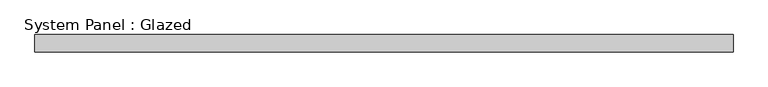
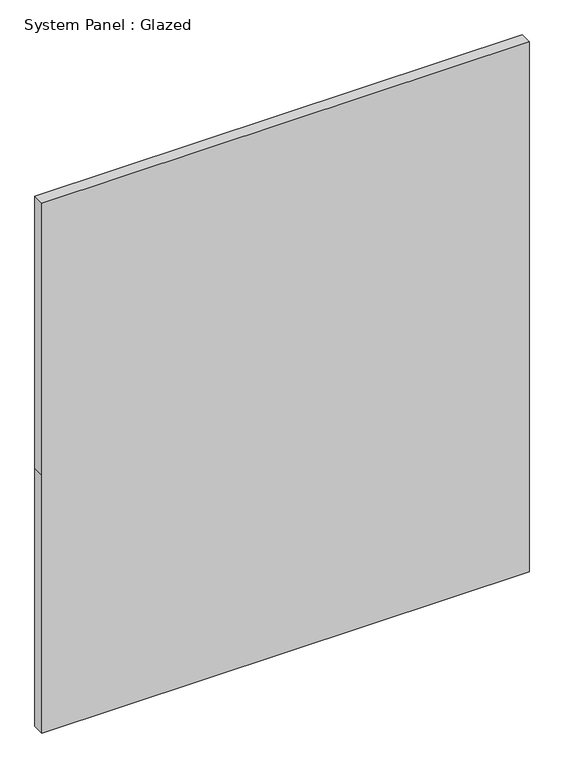
"""IFC4 building model written with IfcOpenShell, lengths in millimetres: plate geometry, System Panel : Glazed."""

import ifcopenshell
import ifcopenshell.guid

model = None  # the IFC model being written
_history = None  # IfcOwnerHistory: only IFC2X3 demands one
_inside = {}  # id of a spatial element -> (the spatial element, [elements in it])
_under = {}  # id of a project, library or spatial element -> (it, [spatial elements below it])
_declared = {}  # id of a project -> (the project, [libraries it declares])
_typed = {}  # id of a type object -> (the type object, [elements of that type])
_made_of = {}  # id of a material, layer set ... -> (it, [elements and type objects made of it])


def new_model(schema):
    """Start an empty IFC model of exactly this schema.

    Asked for "IFC4X3", IfcOpenShell would pick the latest addendum, in which some entities
    have other attributes; the version numbers below select the first issue.
    IFC2X3 requires an IfcOwnerHistory on every rooted entity: one is made here for all.
    """
    global model, _history
    if schema == "IFC4X3":
        model = ifcopenshell.file(schema_version=(4, 3, 0, 0))
    else:
        model = ifcopenshell.file(schema=schema)
    _inside.clear()
    _under.clear()
    _declared.clear()
    _typed.clear()
    _made_of.clear()
    _history = None
    if model.schema == "IFC2X3":
        org = make("IfcOrganization", Name="unknown")
        user = make(
            "IfcPersonAndOrganization",
            ThePerson=make("IfcPerson", FamilyName="unknown"),
            TheOrganization=org,
        )
        app = make(
            "IfcApplication",
            ApplicationDeveloper=org,
            Version="unknown",
            ApplicationFullName="unknown",
            ApplicationIdentifier="unknown",
        )
        _history = make(
            "IfcOwnerHistory",
            OwningUser=user,
            OwningApplication=app,
            ChangeAction="ADDED",
            CreationDate=0,
        )
    return model


def make(cls, **values):
    """One entity of the class cls with the attributes given. An attribute that is None is left unset."""
    return model.create_entity(
        cls, **{name: value for name, value in values.items() if value is not None}
    )


def rooted(cls, **values):
    """An entity with a GlobalId (a new one), such as an element, a storey or a relation."""
    return make(cls, GlobalId=ifcopenshell.guid.new(), OwnerHistory=_history, **values)


def si_unit(unit_type, name, prefix=None):
    """IfcSIUnit, for example si_unit("LENGTHUNIT", "METRE", prefix="MILLI")."""
    return make("IfcSIUnit", UnitType=unit_type, Prefix=prefix, Name=name)


def assignment(units):
    """IfcUnitAssignment: the units of a project."""
    return None if units is None else make("IfcUnitAssignment", Units=units)


def point(xyz):
    """IfcCartesianPoint."""
    return None if xyz is None else make("IfcCartesianPoint", Coordinates=xyz)


def direction(xyz):
    """IfcDirection."""
    return None if xyz is None else make("IfcDirection", DirectionRatios=xyz)


def frame(location, z_axis=None, x_axis=None):
    """IfcAxis2Placement3D, a coordinate frame: its origin and axes. An axis left out is left unset."""
    return make(
        "IfcAxis2Placement3D",
        Location=point(location),
        Axis=direction(z_axis),
        RefDirection=direction(x_axis),
    )


def origin():
    """The frame at (0, 0, 0) with its axes left unset."""
    return frame((0.0, 0.0, 0.0))


def place(relative_to, where):
    """IfcLocalPlacement: puts the frame where relative to a parent placement (None: the world)."""
    return make(
        "IfcLocalPlacement", PlacementRelTo=relative_to, RelativePlacement=where
    )


def context(
    kind, dimensions, precision=None, world=None, true_north=None, identifier=None
):
    """IfcGeometricRepresentationContext, for example the 3D "Model" context."""
    return make(
        "IfcGeometricRepresentationContext",
        ContextIdentifier=identifier,
        ContextType=kind,
        CoordinateSpaceDimension=dimensions,
        Precision=precision,
        WorldCoordinateSystem=world,
        TrueNorth=true_north,
    )


def project(units=None, contexts=None):
    """IfcProject with its units and contexts."""
    return rooted(
        "IfcProject",
        Name="project",
        RepresentationContexts=contexts,
        UnitsInContext=assignment(units),
    )


def spatial(cls, under=None, at=None, **own):
    """A site, building, storey or space (cls), placed at a placement, below another one or the project."""
    s = rooted(cls, ObjectPlacement=at, **own)
    if under is not None:
        _under.setdefault(under.id(), (under, []))[1].append(s)
    return s


def polyline(points):
    """IfcPolyline through the points."""
    return make("IfcPolyline", Points=[point(p) for p in points])


def outline(outer, holes=None, kind="AREA"):
    """IfcArbitraryClosedProfileDef: a profile drawn as a closed curve; with holes, ...WithVoids."""
    if holes is None:
        return make("IfcArbitraryClosedProfileDef", ProfileType=kind, OuterCurve=outer)
    return make(
        "IfcArbitraryProfileDefWithVoids",
        ProfileType=kind,
        OuterCurve=outer,
        InnerCurves=holes,
    )


def extrude(swept, where, along, depth):
    """IfcExtrudedAreaSolid: the profile swept, set in the frame where, extruded along a direction by depth."""
    return make(
        "IfcExtrudedAreaSolid",
        SweptArea=swept,
        Position=where,
        ExtrudedDirection=direction(along),
        Depth=depth,
    )


def shape(context_of_items, identifier, shape_type, items):
    """IfcShapeRepresentation: the items that make up one representation, for example the "Body"."""
    return make(
        "IfcShapeRepresentation",
        ContextOfItems=context_of_items,
        RepresentationIdentifier=identifier,
        RepresentationType=shape_type,
        Items=items,
    )


def source(mapping_origin, context_of_items, identifier, shape_type, items):
    """IfcRepresentationMap: a shape defined once, which mapped items show again and again."""
    return make(
        "IfcRepresentationMap",
        MappingOrigin=mapping_origin,
        MappedRepresentation=shape(context_of_items, identifier, shape_type, items),
    )


def transform(
    local_origin,
    x_axis=None,
    y_axis=None,
    z_axis=None,
    scale=None,
    scale2=None,
    scale3=None,
    uniform=True,
):
    """IfcCartesianTransformationOperator3D, or its non-uniform kind. x_axis, y_axis, z_axis: its Axis1, 2, 3."""
    if uniform:
        return make(
            "IfcCartesianTransformationOperator3D",
            Axis1=direction(x_axis),
            Axis2=direction(y_axis),
            LocalOrigin=point(local_origin),
            Scale=scale,
            Axis3=direction(z_axis),
        )
    return make(
        "IfcCartesianTransformationOperator3DnonUniform",
        Axis1=direction(x_axis),
        Axis2=direction(y_axis),
        LocalOrigin=point(local_origin),
        Scale=scale,
        Axis3=direction(z_axis),
        Scale2=scale2,
        Scale3=scale3,
    )


def mapped(mapping_source, mapping_target):
    """IfcMappedItem: shows the shape of a source again, moved by a transform."""
    return make(
        "IfcMappedItem", MappingSource=mapping_source, MappingTarget=mapping_target
    )


def made_of(thing, what):
    """Note that an element or type object is made of a material, layer set ...; save() writes the relation."""
    if what is not None:
        _made_of.setdefault(what.id(), (what, []))[1].append(thing)
    return thing


def element(
    cls,
    number,
    at=None,
    inside=None,
    cuts=None,
    type_object=None,
    material=None,
    context=None,
    identifier="Body",
    shape_type=None,
    held_by="IfcProductDefinitionShape",
    body=None,
    shapes=None,
    **own,
):
    """One element of the class cls, such as IfcWall. Its Tag is "e" and its number.

    at: its placement. inside: the storey or other place that contains it. cuts: it is an
    opening in that element (IfcRelVoidsElement). A single representation is given by context,
    identifier, shape_type and body (its items); several are given by shapes. held_by: the class
    of the entity that holds the representations. save() writes the other relations.
    """
    e = rooted(cls, Tag="e%d" % number, ObjectPlacement=at, **own)
    if body is not None:
        shapes = [shape(context, identifier, shape_type, body)]
    if shapes is not None:
        e.Representation = make(held_by, Representations=shapes)
    if inside is not None:
        _inside.setdefault(inside.id(), (inside, []))[1].append(e)
    if cuts is not None:
        rooted(
            "IfcRelVoidsElement", RelatingBuildingElement=cuts, RelatedOpeningElement=e
        )
    if type_object is not None:
        _typed.setdefault(type_object.id(), (type_object, []))[1].append(e)
    return made_of(e, material)


def aggregate(whole, parts):
    """IfcRelAggregates: a whole, such as a stair, and the parts it consists of."""
    return rooted("IfcRelAggregates", RelatingObject=whole, RelatedObjects=parts)


def save(model, path):
    """Write the relations noted so far, then the file.

    IfcRelAggregates (storeys below a building ...), IfcRelContainedInSpatialStructure (elements
    in a storey), IfcRelDefinesByType, IfcRelAssociatesMaterial and IfcRelDeclares: one each for
    every whole, place, type object, material and project.
    """
    for whole, parts in _under.values():
        aggregate(whole, parts)
    for where, things in _inside.values():
        rooted(
            "IfcRelContainedInSpatialStructure",
            RelatedElements=things,
            RelatingStructure=where,
        )
    for kind, things in _typed.values():
        rooted("IfcRelDefinesByType", RelatedObjects=things, RelatingType=kind)
    for what, things in _made_of.values():
        rooted("IfcRelAssociatesMaterial", RelatedObjects=things, RelatingMaterial=what)
    for by, libraries in _declared.values():
        rooted("IfcRelDeclares", RelatingContext=by, RelatedDefinitions=libraries)
    model.write(path)


def system_panel_glazed_ee26c616(model_context):
    return source(origin(), model_context, "Body", "SweptSolid", [
        extrude(outline(polyline([(0.0, -516.255), (0.0, 516.255), (577.85, 516.255), (1187.45, 516.255), (1187.45, -516.255), (577.85, -516.255), (0.0, -516.255)])), frame((0.0, -44.45, 0.0), z_axis=(0.0, 1.0, 0.0), x_axis=(0.0, 0.0, 1.0)), (0.0, 0.0, 1.0), 25.4),
    ])


if __name__ == "__main__":
    model = new_model("IFC4")
    model_context = context("Model", 3, world=origin())
    ifc_project = project(units=[si_unit("LENGTHUNIT", "METRE", prefix="MILLI")], contexts=[model_context])
    site = spatial("IfcSite", under=ifc_project)
    building = spatial("IfcBuilding", under=site)
    placement = place(None, origin())
    system_panel_glazed_shape = system_panel_glazed_ee26c616(model_context)
    element("IfcPlate", 1, ObjectType="System Panel : Glazed", at=placement, inside=building, context=model_context, shape_type="MappedRepresentation", body=[
        mapped(system_panel_glazed_shape, transform((0.0, 0.0, 0.0), x_axis=(1.0, 0.0, 0.0), y_axis=(0.0, 1.0, 0.0), z_axis=(0.0, 0.0, 1.0))),
    ])
    save(model, "model.ifc")

# Revit data of these elements
# Element 1 (IfcPlate, "System Panel : Glazed")
#   Materials on its faces: "Glass"
# Materials
#   "Glass": class "Unassigned", colour RGB 0 0 255, transparency 0.75
